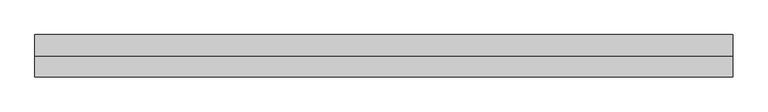
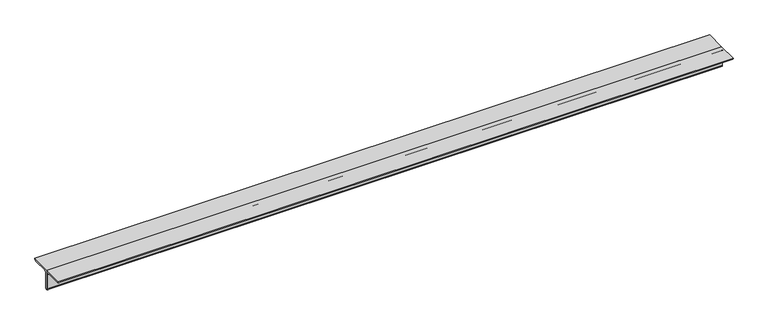
"""IFC4 building model written with IfcOpenShell, lengths in millimetres: member geometry, 0123_Steel Framing_2Ls-KSD3502 : H_SB_AR_S03_2Ls-130x130x12_HBR4."""

from ifc_helpers import new_model, si_unit, point, frame, frame_2d, origin, place, context, project, spatial, polyline, circle_curve, trimmed, segment, composite_curve, outline, extrude, source, transform, mapped, element, save


def member_b79bbe70(model_context):
    return source(origin(), model_context, "Body", "SweptSolid", [
        extrude(outline(composite_curve([segment(polyline([(0.0, 36.4), (130.0, 36.4)]), True, "CONTINUOUS"), segment(trimmed(circle_curve(frame_2d((118.0, 36.4)), 12.0), [point((130.0, 36.4))], [point((118.0, 24.4))], False, "CARTESIAN"), True, "CONTINUOUS"), segment(polyline([(118.0, 24.4), (24.0, 24.4)]), True, "CONTINUOUS"), segment(trimmed(circle_curve(frame_2d((24.0, 12.4)), 12.0), [point((24.0, 24.4))], [point((12.0, 12.4))], True, "CARTESIAN"), True, "CONTINUOUS"), segment(polyline([(12.0, 12.4), (12.0, -81.6)]), True, "CONTINUOUS"), segment(trimmed(circle_curve(frame_2d((0.0, -81.6)), 12.0), [point((12.0, -81.6))], [point((0.0, -93.6))], False, "CARTESIAN"), True, "CONTINUOUS"), segment(polyline([(0.0, -93.6), (0.0, 36.4)]), True, "CONTINUOUS")], self_intersect=False)), frame((-2078.9666667, 0.0, 0.0), z_axis=(1.0, 0.0, 0.0), x_axis=(0.0, 1.0, 0.0)), (0.0, 0.0, 1.0), 4294.8666667),
        extrude(outline(composite_curve([segment(polyline([(0.0, 36.4), (0.0, -93.6)]), True, "CONTINUOUS"), segment(trimmed(circle_curve(frame_2d((0.0, -81.6)), 12.0), [point((0.0, -93.6))], [point((-12.0, -81.6))], False, "CARTESIAN"), True, "CONTINUOUS"), segment(polyline([(-12.0, -81.6), (-12.0, 12.4)]), True, "CONTINUOUS"), segment(trimmed(circle_curve(frame_2d((-24.0, 12.4)), 12.0), [point((-12.0, 12.4))], [point((-24.0, 24.4))], True, "CARTESIAN"), True, "CONTINUOUS"), segment(polyline([(-24.0, 24.4), (-118.0, 24.4)]), True, "CONTINUOUS"), segment(trimmed(circle_curve(frame_2d((-118.0, 36.4)), 12.0), [point((-118.0, 24.4))], [point((-130.0, 36.4))], False, "CARTESIAN"), True, "CONTINUOUS"), segment(polyline([(-130.0, 36.4), (0.0, 36.4)]), True, "CONTINUOUS")], self_intersect=False)), frame((-2078.9666667, 0.0, 0.0), z_axis=(1.0, 0.0, 0.0), x_axis=(0.0, 1.0, 0.0)), (0.0, 0.0, 1.0), 4294.8666667),
    ])


if __name__ == "__main__":
    model = new_model("IFC4")
    model_context = context("Model", 3, world=origin())
    ifc_project = project(units=[si_unit("LENGTHUNIT", "METRE", prefix="MILLI")], contexts=[model_context])
    site = spatial("IfcSite", under=ifc_project)
    building = spatial("IfcBuilding", under=site)
    placement = place(None, origin())
    member_shape = member_b79bbe70(model_context)
    element("IfcMember", 1, ObjectType="0123_Steel Framing_2Ls-KSD3502 : H_SB_AR_S03_2Ls-130x130x12_HBR4", at=placement, inside=building, context=model_context, shape_type="MappedRepresentation", body=[
        mapped(member_shape, transform((0.0, 0.0, 0.0), x_axis=(1.0, 0.0, 0.0), y_axis=(0.0, 1.0, 0.0), z_axis=(0.0, 0.0, 1.0))),
    ])
    save(model, "model.ifc")

# Revit data of these elements
# Type "0123_Steel Framing_2Ls-KSD3502 : H_SB_AR_S03_2Ls-130x130x12_HBR4"
#   Type Mark = "HBR4"
#   Assembly Code = "B10"
#   Legs = "SLBB"
#   W = 8.97
#   Perimeter = 1.04 m²/m
#   Nominal Weight = 46.80 kgf/m
#   Length [instance default] = 1000 mm
#   Space = 0 mm
#   b = 130 mm
#   d = 130 mm
#   t = 12 mm
#   y = 36.4 mm
#   A = 0.005952 m²
#   Structural Material [instance default] = Steel ASTM A36
# Element 1 (IfcMember, "0123_Steel Framing_2Ls-KSD3502 : H_SB_AR_S03_2Ls-130x130x12_HBR4")
#   Materials on its faces: "Steel ASTM A36"
# Materials
#   "Steel ASTM A36": class "Metal", colour RGB 199 199 199, transparency 0, Description = "Structural steel, ASTM A36 Grade B, mill finish", Cost = 0
